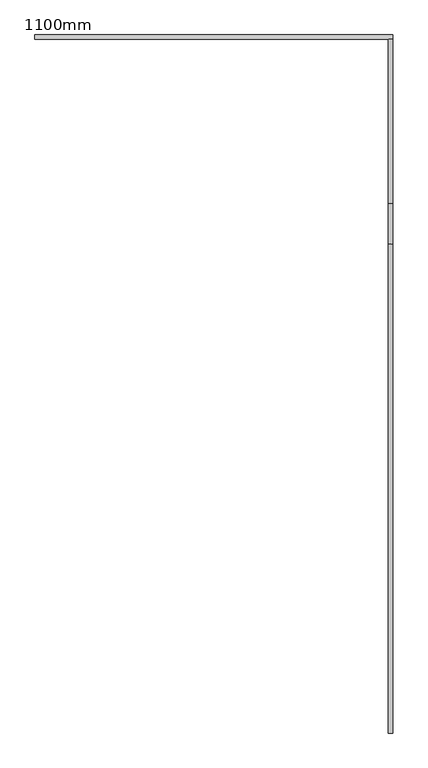
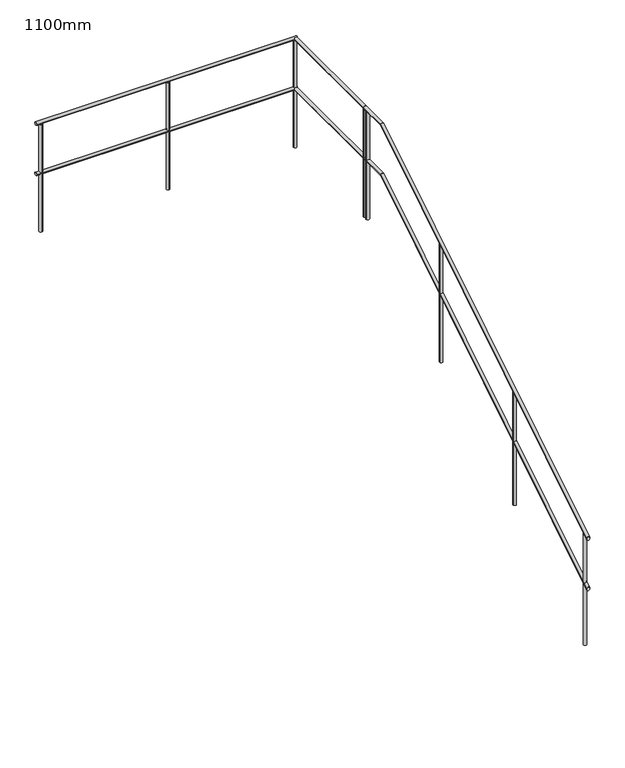
"""IFC4 building model written with IfcOpenShell, lengths in millimetres: railing geometry, 1100mm."""

import ifcopenshell
import ifcopenshell.guid

model = None  # the IFC model being written
_history = None  # IfcOwnerHistory: only IFC2X3 demands one
_inside = {}  # id of a spatial element -> (the spatial element, [elements in it])
_under = {}  # id of a project, library or spatial element -> (it, [spatial elements below it])
_declared = {}  # id of a project -> (the project, [libraries it declares])
_typed = {}  # id of a type object -> (the type object, [elements of that type])
_made_of = {}  # id of a material, layer set ... -> (it, [elements and type objects made of it])


def new_model(schema):
    """Start an empty IFC model of exactly this schema.

    Asked for "IFC4X3", IfcOpenShell would pick the latest addendum, in which some entities
    have other attributes; the version numbers below select the first issue.
    IFC2X3 requires an IfcOwnerHistory on every rooted entity: one is made here for all.
    """
    global model, _history
    if schema == "IFC4X3":
        model = ifcopenshell.file(schema_version=(4, 3, 0, 0))
    else:
        model = ifcopenshell.file(schema=schema)
    _inside.clear()
    _under.clear()
    _declared.clear()
    _typed.clear()
    _made_of.clear()
    _history = None
    if model.schema == "IFC2X3":
        org = make("IfcOrganization", Name="unknown")
        user = make(
            "IfcPersonAndOrganization",
            ThePerson=make("IfcPerson", FamilyName="unknown"),
            TheOrganization=org,
        )
        app = make(
            "IfcApplication",
            ApplicationDeveloper=org,
            Version="unknown",
            ApplicationFullName="unknown",
            ApplicationIdentifier="unknown",
        )
        _history = make(
            "IfcOwnerHistory",
            OwningUser=user,
            OwningApplication=app,
            ChangeAction="ADDED",
            CreationDate=0,
        )
    return model


def make(cls, **values):
    """One entity of the class cls with the attributes given. An attribute that is None is left unset."""
    return model.create_entity(
        cls, **{name: value for name, value in values.items() if value is not None}
    )


def rooted(cls, **values):
    """An entity with a GlobalId (a new one), such as an element, a storey or a relation."""
    return make(cls, GlobalId=ifcopenshell.guid.new(), OwnerHistory=_history, **values)


def si_unit(unit_type, name, prefix=None):
    """IfcSIUnit, for example si_unit("LENGTHUNIT", "METRE", prefix="MILLI")."""
    return make("IfcSIUnit", UnitType=unit_type, Prefix=prefix, Name=name)


def assignment(units):
    """IfcUnitAssignment: the units of a project."""
    return None if units is None else make("IfcUnitAssignment", Units=units)


def point(xyz):
    """IfcCartesianPoint."""
    return None if xyz is None else make("IfcCartesianPoint", Coordinates=xyz)


def direction(xyz):
    """IfcDirection."""
    return None if xyz is None else make("IfcDirection", DirectionRatios=xyz)


def frame(location, z_axis=None, x_axis=None):
    """IfcAxis2Placement3D, a coordinate frame: its origin and axes. An axis left out is left unset."""
    return make(
        "IfcAxis2Placement3D",
        Location=point(location),
        Axis=direction(z_axis),
        RefDirection=direction(x_axis),
    )


def frame_2d(location, x_axis=None):
    """IfcAxis2Placement2D, a coordinate frame in the plane: its origin and x axis."""
    return make(
        "IfcAxis2Placement2D", Location=point(location), RefDirection=direction(x_axis)
    )


def origin():
    """The frame at (0, 0, 0) with its axes left unset."""
    return frame((0.0, 0.0, 0.0))


def place(relative_to, where):
    """IfcLocalPlacement: puts the frame where relative to a parent placement (None: the world)."""
    return make(
        "IfcLocalPlacement", PlacementRelTo=relative_to, RelativePlacement=where
    )


def context(
    kind, dimensions, precision=None, world=None, true_north=None, identifier=None
):
    """IfcGeometricRepresentationContext, for example the 3D "Model" context."""
    return make(
        "IfcGeometricRepresentationContext",
        ContextIdentifier=identifier,
        ContextType=kind,
        CoordinateSpaceDimension=dimensions,
        Precision=precision,
        WorldCoordinateSystem=world,
        TrueNorth=true_north,
    )


def project(units=None, contexts=None):
    """IfcProject with its units and contexts."""
    return rooted(
        "IfcProject",
        Name="project",
        RepresentationContexts=contexts,
        UnitsInContext=assignment(units),
    )


def spatial(cls, under=None, at=None, **own):
    """A site, building, storey or space (cls), placed at a placement, below another one or the project."""
    s = rooted(cls, ObjectPlacement=at, **own)
    if under is not None:
        _under.setdefault(under.id(), (under, []))[1].append(s)
    return s


def circle_curve(where, radius):
    """IfcCircle in the frame where."""
    return make("IfcCircle", Position=where, Radius=radius)


def ellipse_curve(where, semi_axis1, semi_axis2):
    """IfcEllipse in the frame where."""
    return make(
        "IfcEllipse", Position=where, SemiAxis1=semi_axis1, SemiAxis2=semi_axis2
    )


def trimmed(basis, trim1, trim2, sense, master):
    """IfcTrimmedCurve: the piece of a basis curve between two trims."""
    return make(
        "IfcTrimmedCurve",
        BasisCurve=basis,
        Trim1=trim1,
        Trim2=trim2,
        SenseAgreement=sense,
        MasterRepresentation=master,
    )


def segment(curve, same_sense, transition):
    """IfcCompositeCurveSegment."""
    return make(
        "IfcCompositeCurveSegment",
        Transition=transition,
        SameSense=same_sense,
        ParentCurve=curve,
    )


def composite_curve(segments, self_intersect=None):
    """IfcCompositeCurve: segments joined end to end."""
    return make("IfcCompositeCurve", Segments=segments, SelfIntersect=self_intersect)


def outline(outer, holes=None, kind="AREA"):
    """IfcArbitraryClosedProfileDef: a profile drawn as a closed curve; with holes, ...WithVoids."""
    if holes is None:
        return make("IfcArbitraryClosedProfileDef", ProfileType=kind, OuterCurve=outer)
    return make(
        "IfcArbitraryProfileDefWithVoids",
        ProfileType=kind,
        OuterCurve=outer,
        InnerCurves=holes,
    )


def extrude(swept, where, along, depth):
    """IfcExtrudedAreaSolid: the profile swept, set in the frame where, extruded along a direction by depth."""
    return make(
        "IfcExtrudedAreaSolid",
        SweptArea=swept,
        Position=where,
        ExtrudedDirection=direction(along),
        Depth=depth,
    )


def shape(context_of_items, identifier, shape_type, items):
    """IfcShapeRepresentation: the items that make up one representation, for example the "Body"."""
    return make(
        "IfcShapeRepresentation",
        ContextOfItems=context_of_items,
        RepresentationIdentifier=identifier,
        RepresentationType=shape_type,
        Items=items,
    )


def source(mapping_origin, context_of_items, identifier, shape_type, items):
    """IfcRepresentationMap: a shape defined once, which mapped items show again and again."""
    return make(
        "IfcRepresentationMap",
        MappingOrigin=mapping_origin,
        MappedRepresentation=shape(context_of_items, identifier, shape_type, items),
    )


def transform(
    local_origin,
    x_axis=None,
    y_axis=None,
    z_axis=None,
    scale=None,
    scale2=None,
    scale3=None,
    uniform=True,
):
    """IfcCartesianTransformationOperator3D, or its non-uniform kind. x_axis, y_axis, z_axis: its Axis1, 2, 3."""
    if uniform:
        return make(
            "IfcCartesianTransformationOperator3D",
            Axis1=direction(x_axis),
            Axis2=direction(y_axis),
            LocalOrigin=point(local_origin),
            Scale=scale,
            Axis3=direction(z_axis),
        )
    return make(
        "IfcCartesianTransformationOperator3DnonUniform",
        Axis1=direction(x_axis),
        Axis2=direction(y_axis),
        LocalOrigin=point(local_origin),
        Scale=scale,
        Axis3=direction(z_axis),
        Scale2=scale2,
        Scale3=scale3,
    )


def mapped(mapping_source, mapping_target):
    """IfcMappedItem: shows the shape of a source again, moved by a transform."""
    return make(
        "IfcMappedItem", MappingSource=mapping_source, MappingTarget=mapping_target
    )


def made_of(thing, what):
    """Note that an element or type object is made of a material, layer set ...; save() writes the relation."""
    if what is not None:
        _made_of.setdefault(what.id(), (what, []))[1].append(thing)
    return thing


def element(
    cls,
    number,
    at=None,
    inside=None,
    cuts=None,
    type_object=None,
    material=None,
    context=None,
    identifier="Body",
    shape_type=None,
    held_by="IfcProductDefinitionShape",
    body=None,
    shapes=None,
    **own,
):
    """One element of the class cls, such as IfcWall. Its Tag is "e" and its number.

    at: its placement. inside: the storey or other place that contains it. cuts: it is an
    opening in that element (IfcRelVoidsElement). A single representation is given by context,
    identifier, shape_type and body (its items); several are given by shapes. held_by: the class
    of the entity that holds the representations. save() writes the other relations.
    """
    e = rooted(cls, Tag="e%d" % number, ObjectPlacement=at, **own)
    if body is not None:
        shapes = [shape(context, identifier, shape_type, body)]
    if shapes is not None:
        e.Representation = make(held_by, Representations=shapes)
    if inside is not None:
        _inside.setdefault(inside.id(), (inside, []))[1].append(e)
    if cuts is not None:
        rooted(
            "IfcRelVoidsElement", RelatingBuildingElement=cuts, RelatedOpeningElement=e
        )
    if type_object is not None:
        _typed.setdefault(type_object.id(), (type_object, []))[1].append(e)
    return made_of(e, material)


def aggregate(whole, parts):
    """IfcRelAggregates: a whole, such as a stair, and the parts it consists of."""
    return rooted("IfcRelAggregates", RelatingObject=whole, RelatedObjects=parts)


def save(model, path):
    """Write the relations noted so far, then the file.

    IfcRelAggregates (storeys below a building ...), IfcRelContainedInSpatialStructure (elements
    in a storey), IfcRelDefinesByType, IfcRelAssociatesMaterial and IfcRelDeclares: one each for
    every whole, place, type object, material and project.
    """
    for whole, parts in _under.values():
        aggregate(whole, parts)
    for where, things in _inside.values():
        rooted(
            "IfcRelContainedInSpatialStructure",
            RelatedElements=things,
            RelatingStructure=where,
        )
    for kind, things in _typed.values():
        rooted("IfcRelDefinesByType", RelatedObjects=things, RelatingType=kind)
    for what, things in _made_of.values():
        rooted("IfcRelAssociatesMaterial", RelatedObjects=things, RelatingMaterial=what)
    for by, libraries in _declared.values():
        rooted("IfcRelDeclares", RelatingContext=by, RelatedDefinitions=libraries)
    model.write(path)


def plane_surface(at):
    """IfcPlane: the flat surface through the origin of the frame at, square to its z axis."""
    return make("IfcPlane", Position=at)


def cylinder_surface(at, radius):
    """IfcCylindricalSurface: all points at the distance radius from the z axis of the frame at."""
    return make("IfcCylindricalSurface", Position=at, Radius=radius)


def advanced_brep(points, edges, surfaces, faces):
    """IfcAdvancedBrep: a solid bounded by faces that lie on surfaces and meet in shared edges.

    An edge is (start, end): straight between two places in points (the first is 0);
    or (start, end, curve); or (start, end, curve, False) where it runs against its curve.
    A face is (place in surfaces, loops), or (place, loops, False) where it looks against
    its surface's normal. A loop lists edges by number (the first is 1), with a minus sign
    where the edge is run from its end to its start. The first loop is the outer one.
    """
    corners = [point(p) for p in points]
    vertices = [make("IfcVertexPoint", VertexGeometry=c) for c in corners]
    made = []
    for start, end, *more in edges:
        made.append(
            make(
                "IfcEdgeCurve",
                EdgeStart=vertices[start],
                EdgeEnd=vertices[end],
                EdgeGeometry=more[0] if more else make("IfcPolyline", Points=[corners[start], corners[end]]),
                SameSense=more[1] if len(more) > 1 else True,
            )
        )
    hull = []
    for where, loops, *sense in faces:
        bounds = []
        for j, loop in enumerate(loops):
            ring = [make("IfcOrientedEdge", EdgeElement=made[abs(k) - 1], Orientation=k > 0) for k in loop]
            bounds.append(
                make(
                    "IfcFaceOuterBound" if j == 0 else "IfcFaceBound",
                    Bound=make("IfcEdgeLoop", EdgeList=ring),
                    Orientation=True,
                )
            )
        hull.append(make("IfcAdvancedFace", Bounds=bounds, FaceSurface=surfaces[where], SameSense=sense[0] if sense else True))
    return make("IfcAdvancedBrep", Outer=make("IfcClosedShell", CfsFaces=hull))


def railing_1100mm_f57b0715(model_context):
    return source(origin(), model_context, "Body", "SolidModel", [
        advanced_brep(
        [(12685.1052251, 14699.5208589, 456.3396197), (12655.1052251, 14699.5208589, 456.3396197), (12685.1052251, 18339.5208589, 2547.0), (12655.1052251, 18339.5208589, 2547.0), (12685.1052251, 18063.8019306, 2547.0), (12655.1052251, 18063.8019306, 2547.0)],
        [
            (0, 1, ellipse_curve(frame((12670.1052251, 14699.5208589, 456.3396197), z_axis=(0.0, -1.0, 0.0), x_axis=(0.0, 0.0, -1.0)), 17.6603803, 15.0)),
            (1, 0, ellipse_curve(frame((12670.1052251, 14699.5208589, 456.3396197), z_axis=(0.0, -1.0, 0.0), x_axis=(0.0, 0.0, -1.0)), 17.6603803, 15.0)),
            (2, 3, circle_curve(frame((12670.1052251, 18339.5208589, 2547.0), z_axis=(0.0, 1.0, 0.0), x_axis=(-1.0, 0.0, 0.0)), 15.0)),
            (3, 2, circle_curve(frame((12670.1052251, 18339.5208589, 2547.0), z_axis=(0.0, 1.0, 0.0), x_axis=(-1.0, 0.0, 0.0)), 15.0)),
            (0, 4),
            (4, 5, ellipse_curve(frame((12670.1052251, 18063.8019306, 2547.0), z_axis=(0.0, -0.9616025257983003, -0.2744459552959912), x_axis=(0.0, 0.2744459552959914, -0.9616025257983002)), 15.5989607, 15.0)),
            (5, 1),
            (5, 4, ellipse_curve(frame((12670.1052251, 18063.8019306, 2547.0), z_axis=(0.0, -0.9616025257983003, -0.2744459552959912), x_axis=(0.0, 0.2744459552959914, -0.9616025257983002)), 15.5989607, 15.0)),
            (4, 2),
            (3, 5),
        ],
        [
            plane_surface(frame((12670.1052251, 14699.5208589, 474.0), z_axis=(0.0, -1.0, 0.0), x_axis=(0.0, 0.0, 1.0))),
            plane_surface(frame((12670.1052251, 18339.5208589, 2562.0), z_axis=(0.0, 1.0, 0.0), x_axis=(0.0, 0.0, 1.0))),
            cylinder_surface(frame((12670.1052251, 14707.4380966, 461.2596175), z_axis=(0.0, -0.8493588352433417, -0.5278158476155052), x_axis=(-1.0, 0.0, 0.0)), 15.0),
            cylinder_surface(frame((12670.1052251, 18059.5208589, 2547.0), z_axis=(0.0, -1.0, 0.0), x_axis=(-1.0, 0.0, 0.0)), 15.0),
        ],
        [
            (0, [[1, 2]]),
            (1, [[3, 4]]),
            (2, [[-1, 5, 6, 7]]),
            (2, [[-2, -7, 8, -5]]),
            (3, [[-6, 9, -4, 10]]),
            (3, [[-8, -10, -3, -9]]),
        ],
    ),
        advanced_brep(
        [(12685.1052251, 18339.5208589, 2547.0), (12655.1052251, 18339.5208589, 2547.0), (12685.1052251, 19469.5208589, 2547.0), (12655.1052251, 19469.5208589, 2547.0)],
        [
            (0, 1, circle_curve(frame((12670.1052251, 18339.5208589, 2547.0), z_axis=(0.0, -1.0, 0.0), x_axis=(-1.0, 0.0, 0.0)), 15.0)),
            (1, 0, circle_curve(frame((12670.1052251, 18339.5208589, 2547.0), z_axis=(0.0, -1.0, 0.0), x_axis=(-1.0, 0.0, 0.0)), 15.0)),
            (2, 3, circle_curve(frame((12670.1052251, 19469.5208589, 2547.0), z_axis=(0.0, 1.0, 0.0), x_axis=(-1.0, 0.0, 0.0)), 15.0)),
            (3, 2, circle_curve(frame((12670.1052251, 19469.5208589, 2547.0), z_axis=(0.0, 1.0, 0.0), x_axis=(-1.0, 0.0, 0.0)), 15.0)),
            (0, 2),
            (3, 1),
        ],
        [
            plane_surface(frame((12670.1052251, 18339.5208589, 2562.0), z_axis=(0.0, -1.0, 0.0), x_axis=(0.0, 0.0, 1.0))),
            plane_surface(frame((12670.1052251, 19469.5208589, 2562.0), z_axis=(0.0, 1.0, 0.0), x_axis=(0.0, 0.0, 1.0))),
            cylinder_surface(frame((12670.1052251, 18339.5208589, 2547.0), z_axis=(0.0, -1.0, 0.0), x_axis=(-1.0, 0.0, 0.0)), 15.0),
        ],
        [
            (0, [[1, 2]]),
            (1, [[3, 4]]),
            (2, [[-1, 5, -4, 6]]),
            (2, [[-2, -6, -3, -5]]),
        ],
    ),
        advanced_brep(
        [(12685.1052251, 19499.5208589, 2547.0), (12685.1052251, 19469.5208589, 2547.0), (10225.1052251, 19499.5208589, 2547.0), (10225.1052251, 19469.5208589, 2547.0)],
        [
            (0, 1, circle_curve(frame((12685.1052251, 19484.5208589, 2547.0), z_axis=(1.0, 0.0, 0.0), x_axis=(0.0, -1.0, 0.0)), 15.0)),
            (1, 0, circle_curve(frame((12685.1052251, 19484.5208589, 2547.0), z_axis=(1.0, 0.0, 0.0), x_axis=(0.0, -1.0, 0.0)), 15.0)),
            (2, 3, circle_curve(frame((10225.1052251, 19484.5208589, 2547.0), z_axis=(-1.0, 0.0, 0.0), x_axis=(0.0, -1.0, 0.0)), 15.0)),
            (3, 2, circle_curve(frame((10225.1052251, 19484.5208589, 2547.0), z_axis=(-1.0, 0.0, 0.0), x_axis=(0.0, -1.0, 0.0)), 15.0)),
            (0, 2),
            (3, 1),
        ],
        [
            plane_surface(frame((12685.1052251, 19484.5208589, 2562.0), z_axis=(1.0, 0.0, 0.0), x_axis=(0.0, -1.0, 0.0))),
            plane_surface(frame((10225.1052251, 19484.5208589, 2562.0), z_axis=(-1.0, 0.0, 0.0), x_axis=(0.0, -1.0, 0.0))),
            cylinder_surface(frame((12685.1052251, 19484.5208589, 2547.0), z_axis=(1.0, 0.0, 0.0), x_axis=(0.0, -1.0, 0.0)), 15.0),
        ],
        [
            (0, [[1, 2]]),
            (1, [[3, 4]]),
            (2, [[-1, 5, -4, 6]]),
            (2, [[-2, -6, -3, -5]]),
        ],
    ),
        advanced_brep(
        [(12685.1052251, 14699.5208589, 956.3396197), (12655.1052251, 14699.5208589, 956.3396197), (12685.1052251, 18063.8019306, 3047.0), (12655.1052251, 18063.8019306, 3047.0), (12685.1052251, 18339.5208589, 3047.0), (12655.1052251, 18339.5208589, 3047.0)],
        [
            (0, 1, ellipse_curve(frame((12670.1052251, 14699.5208589, 956.3396197), z_axis=(0.0, -1.0, 0.0), x_axis=(0.0, 0.0, -1.0)), 17.6603803, 15.0)),
            (1, 0, ellipse_curve(frame((12670.1052251, 14699.5208589, 956.3396197), z_axis=(0.0, -1.0, 0.0), x_axis=(0.0, 0.0, -1.0)), 17.6603803, 15.0)),
            (0, 2),
            (2, 3, ellipse_curve(frame((12670.1052251, 18063.8019306, 3047.0), z_axis=(0.0, -0.9616025257983003, -0.2744459552959912), x_axis=(0.0, 0.2744459552959914, -0.9616025257983002)), 15.5989607, 15.0)),
            (3, 1),
            (3, 2, ellipse_curve(frame((12670.1052251, 18063.8019306, 3047.0), z_axis=(0.0, -0.9616025257983003, -0.2744459552959912), x_axis=(0.0, 0.2744459552959914, -0.9616025257983002)), 15.5989607, 15.0)),
            (4, 5, circle_curve(frame((12670.1052251, 18339.5208589, 3047.0), z_axis=(0.0, 1.0, 0.0), x_axis=(-1.0, 0.0, 0.0)), 15.0)),
            (5, 4, circle_curve(frame((12670.1052251, 18339.5208589, 3047.0), z_axis=(0.0, 1.0, 0.0), x_axis=(-1.0, 0.0, 0.0)), 15.0)),
            (2, 4),
            (5, 3),
        ],
        [
            plane_surface(frame((12670.1052251, 14699.5208589, 974.0), z_axis=(0.0, -1.0, 0.0), x_axis=(0.0, 0.0, 1.0))),
            cylinder_surface(frame((12670.1052251, 14707.4380966, 961.2596175), z_axis=(0.0, -0.8493588352433417, -0.5278158476155052), x_axis=(-1.0, 0.0, 0.0)), 15.0),
            plane_surface(frame((12670.1052251, 18339.5208589, 3062.0), z_axis=(0.0, 1.0, 0.0), x_axis=(0.0, 0.0, 1.0))),
            cylinder_surface(frame((12670.1052251, 18059.5208589, 3047.0), z_axis=(0.0, -1.0, 0.0), x_axis=(-1.0, 0.0, 0.0)), 15.0),
        ],
        [
            (0, [[1, 2]]),
            (1, [[-1, 3, 4, 5]]),
            (1, [[-2, -5, 6, -3]]),
            (2, [[7, 8]]),
            (3, [[-4, 9, -8, 10]]),
            (3, [[-6, -10, -7, -9]]),
        ],
    ),
        advanced_brep(
        [(12685.1052251, 18339.5208589, 3047.0), (12655.1052251, 18339.5208589, 3047.0), (12685.1052251, 19469.5208589, 3047.0), (12655.1052251, 19469.5208589, 3047.0)],
        [
            (0, 1, circle_curve(frame((12670.1052251, 18339.5208589, 3047.0), z_axis=(0.0, -1.0, 0.0), x_axis=(-1.0, 0.0, 0.0)), 15.0)),
            (1, 0, circle_curve(frame((12670.1052251, 18339.5208589, 3047.0), z_axis=(0.0, -1.0, 0.0), x_axis=(-1.0, 0.0, 0.0)), 15.0)),
            (2, 3, circle_curve(frame((12670.1052251, 19469.5208589, 3047.0), z_axis=(0.0, 1.0, 0.0), x_axis=(-1.0, 0.0, 0.0)), 15.0)),
            (3, 2, circle_curve(frame((12670.1052251, 19469.5208589, 3047.0), z_axis=(0.0, 1.0, 0.0), x_axis=(-1.0, 0.0, 0.0)), 15.0)),
            (0, 2),
            (3, 1),
        ],
        [
            plane_surface(frame((12670.1052251, 18339.5208589, 3062.0), z_axis=(0.0, -1.0, 0.0), x_axis=(0.0, 0.0, 1.0))),
            plane_surface(frame((12670.1052251, 19469.5208589, 3062.0), z_axis=(0.0, 1.0, 0.0), x_axis=(0.0, 0.0, 1.0))),
            cylinder_surface(frame((12670.1052251, 18339.5208589, 3047.0), z_axis=(0.0, -1.0, 0.0), x_axis=(-1.0, 0.0, 0.0)), 15.0),
        ],
        [
            (0, [[1, 2]]),
            (1, [[3, 4]]),
            (2, [[-1, 5, -4, 6]]),
            (2, [[-2, -6, -3, -5]]),
        ],
    ),
        advanced_brep(
        [(12685.1052251, 19499.5208589, 3047.0), (12685.1052251, 19469.5208589, 3047.0), (10225.1052251, 19499.5208589, 3047.0), (10225.1052251, 19469.5208589, 3047.0)],
        [
            (0, 1, circle_curve(frame((12685.1052251, 19484.5208589, 3047.0), z_axis=(1.0, 0.0, 0.0), x_axis=(0.0, -1.0, 0.0)), 15.0)),
            (1, 0, circle_curve(frame((12685.1052251, 19484.5208589, 3047.0), z_axis=(1.0, 0.0, 0.0), x_axis=(0.0, -1.0, 0.0)), 15.0)),
            (2, 3, circle_curve(frame((10225.1052251, 19484.5208589, 3047.0), z_axis=(-1.0, 0.0, 0.0), x_axis=(0.0, -1.0, 0.0)), 15.0)),
            (3, 2, circle_curve(frame((10225.1052251, 19484.5208589, 3047.0), z_axis=(-1.0, 0.0, 0.0), x_axis=(0.0, -1.0, 0.0)), 15.0)),
            (0, 2),
            (3, 1),
        ],
        [
            plane_surface(frame((12685.1052251, 19484.5208589, 3062.0), z_axis=(1.0, 0.0, 0.0), x_axis=(0.0, -1.0, 0.0))),
            plane_surface(frame((10225.1052251, 19484.5208589, 3062.0), z_axis=(-1.0, 0.0, 0.0), x_axis=(0.0, -1.0, 0.0))),
            cylinder_surface(frame((12685.1052251, 19484.5208589, 3047.0), z_axis=(1.0, 0.0, 0.0), x_axis=(0.0, -1.0, 0.0)), 15.0),
        ],
        [
            (0, [[1, 2]]),
            (1, [[3, 4]]),
            (2, [[-1, 5, -4, 6]]),
            (2, [[-2, -6, -3, -5]]),
        ],
    ),
        extrude(outline(composite_curve([segment(trimmed(circle_curve(frame_2d((10270.1052251, 19484.5208589)), 15.0), [point((10270.1052251, 19469.5208589))], [point((10270.1052251, 19499.5208589))], False, "CARTESIAN"), True, "CONTINUOUS"), segment(trimmed(circle_curve(frame_2d((10270.1052251, 19484.5208589)), 15.0), [point((10270.1052251, 19499.5208589))], [point((10270.1052251, 19469.5208589))], False, "CARTESIAN"), True, "CONTINUOUS")], self_intersect=False)), frame((0.0, 0.0, 1962.0), z_axis=(0.0, 0.0, 1.0), x_axis=(1.0, 0.0, 0.0)), (0.0, 0.0, 1.0), 1070.0),
        extrude(outline(composite_curve([segment(trimmed(circle_curve(frame_2d((11470.1052251, 19484.5208589)), 15.0), [point((11470.1052251, 19469.5208589))], [point((11470.1052251, 19499.5208589))], False, "CARTESIAN"), True, "CONTINUOUS"), segment(trimmed(circle_curve(frame_2d((11470.1052251, 19484.5208589)), 15.0), [point((11470.1052251, 19499.5208589))], [point((11470.1052251, 19469.5208589))], False, "CARTESIAN"), True, "CONTINUOUS")], self_intersect=False)), frame((0.0, 0.0, 1962.0), z_axis=(0.0, 0.0, 1.0), x_axis=(1.0, 0.0, 0.0)), (0.0, 0.0, 1.0), 1070.0),
        extrude(outline(composite_curve([segment(trimmed(circle_curve(frame_2d((12670.1052251, 18299.5208589)), 15.0), [point((12655.1052251, 18299.5208589))], [point((12685.1052251, 18299.5208589))], False, "CARTESIAN"), True, "CONTINUOUS"), segment(trimmed(circle_curve(frame_2d((12670.1052251, 18299.5208589)), 15.0), [point((12685.1052251, 18299.5208589))], [point((12655.1052251, 18299.5208589))], False, "CARTESIAN"), True, "CONTINUOUS")], self_intersect=False)), frame((0.0, 0.0, 1962.0), z_axis=(0.0, 0.0, 1.0), x_axis=(1.0, 0.0, 0.0)), (0.0, 0.0, 1.0), 1070.0),
        extrude(outline(composite_curve([segment(trimmed(circle_curve(frame_2d((12670.1052251, 17099.5208589)), 15.0), [point((12655.1052251, 17099.5208589))], [point((12685.1052251, 17099.5208589))], False, "CARTESIAN"), True, "CONTINUOUS"), segment(trimmed(circle_curve(frame_2d((12670.1052251, 17099.5208589)), 15.0), [point((12685.1052251, 17099.5208589))], [point((12655.1052251, 17099.5208589))], False, "CARTESIAN"), True, "CONTINUOUS")], self_intersect=False)), frame((0.0, 0.0, 1266.0), z_axis=(0.0, 0.0, 1.0), x_axis=(1.0, 0.0, 0.0)), (0.0, 0.0, 1.0), 1169.4285714),
        extrude(outline(composite_curve([segment(trimmed(circle_curve(frame_2d((12670.1052251, 15899.5208589)), 15.0), [point((12655.1052251, 15899.5208589))], [point((12685.1052251, 15899.5208589))], False, "CARTESIAN"), True, "CONTINUOUS"), segment(trimmed(circle_curve(frame_2d((12670.1052251, 15899.5208589)), 15.0), [point((12685.1052251, 15899.5208589))], [point((12655.1052251, 15899.5208589))], False, "CARTESIAN"), True, "CONTINUOUS")], self_intersect=False)), frame((0.0, 0.0, 570.0), z_axis=(0.0, 0.0, 1.0), x_axis=(1.0, 0.0, 0.0)), (0.0, 0.0, 1.0), 1119.7142857),
        extrude(outline(composite_curve([segment(trimmed(circle_curve(frame_2d((12670.1052251, 19484.5208589)), 15.0), [point((12655.1052251, 19484.5208589))], [point((12685.1052251, 19484.5208589))], False, "CARTESIAN"), True, "CONTINUOUS"), segment(trimmed(circle_curve(frame_2d((12670.1052251, 19484.5208589)), 15.0), [point((12685.1052251, 19484.5208589))], [point((12655.1052251, 19484.5208589))], False, "CARTESIAN"), True, "CONTINUOUS")], self_intersect=False)), frame((0.0, 0.0, 1962.0), z_axis=(0.0, 0.0, 1.0), x_axis=(1.0, 0.0, 0.0)), (0.0, 0.0, 1.0), 1070.0),
        extrude(outline(composite_curve([segment(trimmed(circle_curve(frame_2d((12670.1052251, 18339.5208589)), 15.0), [point((12655.1052251, 18339.5208589))], [point((12685.1052251, 18339.5208589))], False, "CARTESIAN"), True, "CONTINUOUS"), segment(trimmed(circle_curve(frame_2d((12670.1052251, 18339.5208589)), 15.0), [point((12685.1052251, 18339.5208589))], [point((12655.1052251, 18339.5208589))], False, "CARTESIAN"), True, "CONTINUOUS")], self_intersect=False)), frame((0.0, 0.0, 1962.0), z_axis=(0.0, 0.0, 1.0), x_axis=(1.0, 0.0, 0.0)), (0.0, 0.0, 1.0), 1070.0),
        extrude(outline(composite_curve([segment(trimmed(circle_curve(frame_2d((10275.1052251, 19484.5208589)), 15.0), [point((10275.1052251, 19469.5208589))], [point((10275.1052251, 19499.5208589))], False, "CARTESIAN"), True, "CONTINUOUS"), segment(trimmed(circle_curve(frame_2d((10275.1052251, 19484.5208589)), 15.0), [point((10275.1052251, 19499.5208589))], [point((10275.1052251, 19469.5208589))], False, "CARTESIAN"), True, "CONTINUOUS")], self_intersect=False)), frame((0.0, 0.0, 1962.0), z_axis=(0.0, 0.0, 1.0), x_axis=(1.0, 0.0, 0.0)), (0.0, 0.0, 1.0), 1070.0),
        extrude(outline(composite_curve([segment(trimmed(circle_curve(frame_2d((12670.1052251, 14749.5208589)), 15.0), [point((12655.1052251, 14749.5208589))], [point((12685.1052251, 14749.5208589))], False, "CARTESIAN"), True, "CONTINUOUS"), segment(trimmed(circle_curve(frame_2d((12670.1052251, 14749.5208589)), 15.0), [point((12685.1052251, 14749.5208589))], [point((12655.1052251, 14749.5208589))], False, "CARTESIAN"), True, "CONTINUOUS")], self_intersect=False)), frame((0.0, 0.0, -126.0), z_axis=(0.0, 0.0, 1.0), x_axis=(1.0, 0.0, 0.0)), (0.0, 0.0, 1.0), 1101.0714286),
    ])


if __name__ == "__main__":
    model = new_model("IFC4")
    model_context = context("Model", 3, world=origin())
    ifc_project = project(units=[si_unit("LENGTHUNIT", "METRE", prefix="MILLI")], contexts=[model_context])
    site = spatial("IfcSite", under=ifc_project)
    building = spatial("IfcBuilding", under=site)
    placement = place(None, origin())
    railing_1100mm_shape = railing_1100mm_f57b0715(model_context)
    element("IfcRailing", 1, ObjectType="1100mm", at=placement, inside=building, context=model_context, shape_type="MappedRepresentation", body=[
        mapped(railing_1100mm_shape, transform((0.0, 0.0, 0.0), x_axis=(1.0, 0.0, 0.0), y_axis=(0.0, 1.0, 0.0), z_axis=(0.0, 0.0, 1.0))),
    ])
    save(model, "model.ifc")
